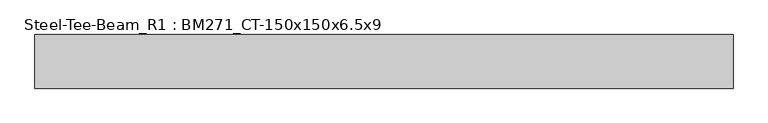
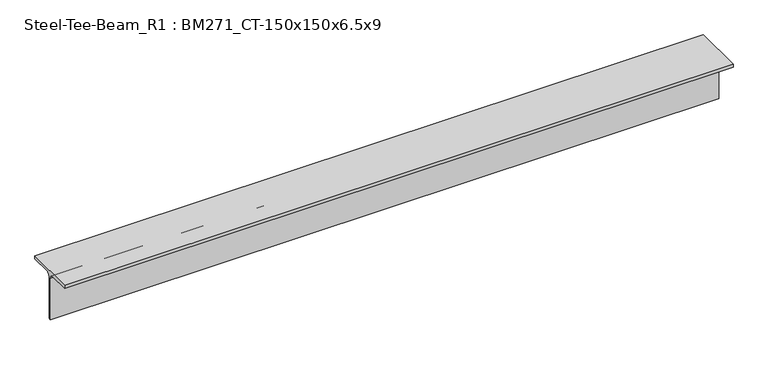
"""IFC4 building model written with IfcOpenShell, lengths in millimetres: member geometry, Steel-Tee-Beam_R1 : BM271_CT-150x150x6.5x9."""

from ifc_helpers import new_model, si_unit, point, frame, frame_2d, origin, place, context, project, spatial, polyline, circle_curve, trimmed, segment, composite_curve, outline, extrude, source, transform, mapped, element, save


def steel_tee_beam_r1_bm271_ct_150x150x6_5x9_3f4c891e(model_context):
    return source(origin(), model_context, "Body", "SweptSolid", [
        extrude(outline(composite_curve([segment(polyline([(75.0, 75.0), (75.0, 66.0), (16.25, 66.0)]), True, "CONTINUOUS"), segment(trimmed(circle_curve(frame_2d((16.25, 53.0)), 13.0), [point((16.25, 66.0))], [point((3.25, 53.0))], True, "CARTESIAN"), True, "CONTINUOUS"), segment(polyline([(3.25, 53.0), (3.25, -75.0), (-3.25, -75.0), (-3.25, 53.0)]), True, "CONTINUOUS"), segment(trimmed(circle_curve(frame_2d((-16.25, 53.0)), 13.0), [point((-3.25, 53.0))], [point((-16.25, 66.0))], True, "CARTESIAN"), True, "CONTINUOUS"), segment(polyline([(-16.25, 66.0), (-75.0, 66.0), (-75.0, 75.0), (75.0, 75.0)]), True, "CONTINUOUS")], self_intersect=False)), frame((-983.9814396, 0.0, 0.0), z_axis=(1.0, 0.0, 0.0), x_axis=(0.0, 1.0, 0.0)), (0.0, 0.0, 1.0), 1951.2705213),
    ])


if __name__ == "__main__":
    model = new_model("IFC4")
    model_context = context("Model", 3, world=origin())
    ifc_project = project(units=[si_unit("LENGTHUNIT", "METRE", prefix="MILLI")], contexts=[model_context])
    site = spatial("IfcSite", under=ifc_project)
    building = spatial("IfcBuilding", under=site)
    placement = place(None, origin())
    steel_tee_beam_r1_bm271_ct_150x150x6_5x9_shape = steel_tee_beam_r1_bm271_ct_150x150x6_5x9_3f4c891e(model_context)
    element("IfcMember", 1, ObjectType="Steel-Tee-Beam_R1 : BM271_CT-150x150x6.5x9", at=placement, inside=building, context=model_context, shape_type="MappedRepresentation", body=[
        mapped(steel_tee_beam_r1_bm271_ct_150x150x6_5x9_shape, transform((0.0, 0.0, 0.0), x_axis=(1.0, 0.0, 0.0), y_axis=(0.0, 1.0, 0.0), z_axis=(0.0, 0.0, 1.0))),
    ])
    save(model, "model.ifc")

# Revit data of these elements
# Type "Steel-Tee-Beam_R1 : BM271_CT-150x150x6.5x9"
#   Keynote = "CT-150x150x6.5x9"
#   Surface Area = 0.588841 m²/m
#   Section Area = 23.3904 cm²
#   Mass per Unit Length = 18.3614 kg/m
#   Length [instance default] = 1.5240 m
#   bf = 0.1500 m
#   d = 0.1500 m
#   k = 0.0220 m
#   r = 0.0130 m
#   tf = 0.0090 m
#   tw = 0.0065 m
#   hec_material4 [instance default] = none
#   hec_material3 [instance default] = none
#   hec_material2 [instance default] = none
#   hec_material1 [instance default] = none
#   Structural Material [instance default] = Steel, 45-345
#   Assembly Code = ""
# Element 1 (IfcMember, "Steel-Tee-Beam_R1 : BM271_CT-150x150x6.5x9")
#   Structural Material = none
# Materials
#   "Steel, 45-345": class "Metal", colour RGB 189 187 185, transparency 0, Description = "Steel 345 MPa", Cost = 0
